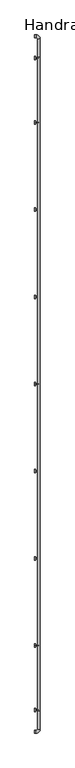
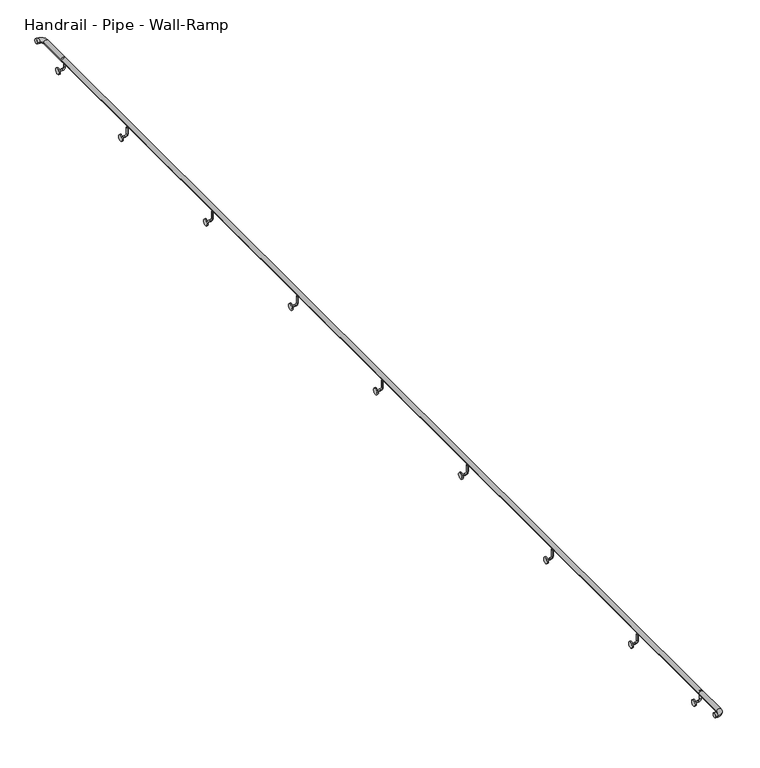
"""IFC4 building model written with IfcOpenShell, lengths in millimetres: railing geometry, Handrail - Pipe - Wall-Ramp."""

from ifc_helpers import new_model, si_unit, point, frame, frame_2d, origin, place, context, project, spatial, circle_curve, ellipse_curve, trimmed, segment, composite_curve, outline, extrude, source, transform, mapped, element, save
from ifc_brep_helpers import plane_surface, cylinder_surface, revolved_surface, advanced_brep


def handrail_pipe_wall_ramp_f1563d15(model_context):
    return source(origin(), model_context, "Body", "SolidModel", [
        extrude(outline(composite_curve([segment(trimmed(circle_curve(frame_2d((895.35, -6025.1478678)), 19.05), [point((895.35, -6006.0978678))], [point((895.35, -6044.1978678))], False, "CARTESIAN"), True, "CONTINUOUS"), segment(trimmed(circle_curve(frame_2d((895.35, -6025.1478678)), 19.05), [point((895.35, -6044.1978678))], [point((895.35, -6006.0978678))], False, "CARTESIAN"), True, "CONTINUOUS")], self_intersect=False)), frame((0.0, -14489.4143828, 0.0), z_axis=(0.0, 1.0, 0.0), x_axis=(0.0, 0.0, 1.0)), (0.0, 0.0, 1.0), 9144.0),
        advanced_brep(
        [(-6025.1478678, -13568.6643828, 857.25), (-6025.1478678, -13581.3643828, 857.25), (-6025.1478678, -13568.6643828, 800.1), (-6025.1478678, -13581.3643828, 800.1), (-6044.1978678, -13581.3643828, 781.05), (-6044.1978678, -13568.6643828, 781.05), (-6072.7728678, -13568.6643828, 781.05), (-6072.7728678, -13581.3643828, 781.05)],
        [
            (0, 1, circle_curve(frame((-6025.1478678, -13575.0143828, 857.25), z_axis=(0.0, 0.0, 1.0), x_axis=(0.0, -1.0, 0.0)), 6.35)),
            (1, 0, circle_curve(frame((-6025.1478678, -13575.0143828, 857.25), z_axis=(0.0, 0.0, 1.0), x_axis=(0.0, -1.0, 0.0)), 6.35)),
            (0, 2),
            (2, 3, circle_curve(frame((-6025.1478678, -13575.0143828, 800.1), z_axis=(0.0, 0.0, 1.0), x_axis=(0.0, -1.0, 0.0)), 6.35)),
            (3, 1),
            (3, 2, circle_curve(frame((-6025.1478678, -13575.0143828, 800.1), z_axis=(0.0, 0.0, 1.0), x_axis=(0.0, -1.0, 0.0)), 6.35)),
            (4, 3, circle_curve(frame((-6044.1978678, -13581.3643828, 800.1), z_axis=(0.0, -1.0, 0.0), x_axis=(1.0, 0.0, 0.0)), 19.05)),
            (2, 5, circle_curve(frame((-6044.1978678, -13568.6643828, 800.1), z_axis=(0.0, 1.0, 0.0), x_axis=(1.0, 0.0, 0.0)), 19.05)),
            (5, 4, circle_curve(frame((-6044.1978678, -13575.0143828, 781.05), z_axis=(1.0, 0.0, 0.0), x_axis=(0.0, -1.0, 0.0)), 6.35)),
            (4, 5, circle_curve(frame((-6044.1978678, -13575.0143828, 781.05), z_axis=(1.0, 0.0, 0.0), x_axis=(0.0, -1.0, 0.0)), 6.35)),
            (6, 7, circle_curve(frame((-6072.7728678, -13575.0143828, 781.05), z_axis=(-1.0, 0.0, 0.0), x_axis=(0.0, -1.0, 0.0)), 6.35)),
            (7, 6, circle_curve(frame((-6072.7728678, -13575.0143828, 781.05), z_axis=(-1.0, 0.0, 0.0), x_axis=(0.0, -1.0, 0.0)), 6.35)),
            (5, 6),
            (7, 4),
        ],
        [
            plane_surface(frame((-6025.1478678, -13581.3643828, 857.25), z_axis=(0.0, 0.0, 1.0), x_axis=(-1.0, 0.0, 0.0))),
            cylinder_surface(frame((-6025.1478678, -13575.0143828, 857.25), z_axis=(0.0, 0.0, 1.0), x_axis=(0.0, -1.0, 0.0)), 6.35),
            revolved_surface(trimmed(ellipse_curve(frame((-6025.1478678, -13575.0143828, 800.1), z_axis=(0.0, 0.0, 1.0), x_axis=(0.0, -1.0, 0.0)), 6.35, 6.35), [point((-6025.1478678, -13568.6643828, 800.1))], [point((-6025.1478678, -13581.3643828, 800.1))], True, "CARTESIAN"), (-6044.1978678, -13575.0143828, 800.1), (0.0, 1.0, 0.0)),
            revolved_surface(trimmed(ellipse_curve(frame((-6025.1478678, -13575.0143828, 800.1), z_axis=(0.0, 0.0, 1.0), x_axis=(0.0, -1.0, 0.0)), 6.35, 6.35), [point((-6025.1478678, -13581.3643828, 800.1))], [point((-6025.1478678, -13568.6643828, 800.1))], True, "CARTESIAN"), (-6044.1978678, -13575.0143828, 800.1), (0.0, 1.0, 0.0)),
            plane_surface(frame((-6072.7728678, -13575.0143828, 774.7), z_axis=(-1.0, 0.0, 0.0), x_axis=(0.0, -1.0, 0.0))),
            cylinder_surface(frame((-6044.1978678, -13575.0143828, 781.05), z_axis=(1.0, 0.0, 0.0), x_axis=(0.0, -1.0, 0.0)), 6.35),
        ],
        [
            (0, [[1, 2]]),
            (1, [[-1, 3, 4, 5]]),
            (1, [[-2, -5, 6, -3]]),
            (2, [[7, -4, 8, 9]]),
            (3, [[-8, -6, -7, 10]]),
            (4, [[11, 12]]),
            (5, [[-9, 13, -12, 14]]),
            (5, [[-10, -14, -11, -13]]),
        ],
    ),
        extrude(outline(composite_curve([segment(trimmed(circle_curve(frame_2d((-13575.0143828, 781.05)), 25.4), [point((-13600.4143828, 781.05))], [point((-13549.6143828, 781.05))], False, "CARTESIAN"), True, "CONTINUOUS"), segment(trimmed(circle_curve(frame_2d((-13575.0143828, 781.05)), 25.4), [point((-13549.6143828, 781.05))], [point((-13600.4143828, 781.05))], False, "CARTESIAN"), True, "CONTINUOUS")], self_intersect=False)), frame((-6082.2978678, 0.0, 0.0), z_axis=(1.0, 0.0, 0.0), x_axis=(0.0, 1.0, 0.0)), (0.0, 0.0, 1.0), 9.525),
        advanced_brep(
        [(-6025.1478678, -12349.4643828, 857.25), (-6025.1478678, -12362.1643828, 857.25), (-6025.1478678, -12349.4643828, 800.1), (-6025.1478678, -12362.1643828, 800.1), (-6044.1978678, -12362.1643828, 781.05), (-6044.1978678, -12349.4643828, 781.05), (-6072.7728678, -12349.4643828, 781.05), (-6072.7728678, -12362.1643828, 781.05)],
        [
            (0, 1, circle_curve(frame((-6025.1478678, -12355.8143828, 857.25), z_axis=(0.0, 0.0, 1.0), x_axis=(0.0, -1.0, 0.0)), 6.35)),
            (1, 0, circle_curve(frame((-6025.1478678, -12355.8143828, 857.25), z_axis=(0.0, 0.0, 1.0), x_axis=(0.0, -1.0, 0.0)), 6.35)),
            (0, 2),
            (2, 3, circle_curve(frame((-6025.1478678, -12355.8143828, 800.1), z_axis=(0.0, 0.0, 1.0), x_axis=(0.0, -1.0, 0.0)), 6.35)),
            (3, 1),
            (3, 2, circle_curve(frame((-6025.1478678, -12355.8143828, 800.1), z_axis=(0.0, 0.0, 1.0), x_axis=(0.0, -1.0, 0.0)), 6.35)),
            (4, 3, circle_curve(frame((-6044.1978678, -12362.1643828, 800.1), z_axis=(0.0, -1.0, 0.0), x_axis=(1.0, 0.0, 0.0)), 19.05)),
            (2, 5, circle_curve(frame((-6044.1978678, -12349.4643828, 800.1), z_axis=(0.0, 1.0, 0.0), x_axis=(1.0, 0.0, 0.0)), 19.05)),
            (5, 4, circle_curve(frame((-6044.1978678, -12355.8143828, 781.05), z_axis=(1.0, 0.0, 0.0), x_axis=(0.0, -1.0, 0.0)), 6.35)),
            (4, 5, circle_curve(frame((-6044.1978678, -12355.8143828, 781.05), z_axis=(1.0, 0.0, 0.0), x_axis=(0.0, -1.0, 0.0)), 6.35)),
            (6, 7, circle_curve(frame((-6072.7728678, -12355.8143828, 781.05), z_axis=(-1.0, 0.0, 0.0), x_axis=(0.0, -1.0, 0.0)), 6.35)),
            (7, 6, circle_curve(frame((-6072.7728678, -12355.8143828, 781.05), z_axis=(-1.0, 0.0, 0.0), x_axis=(0.0, -1.0, 0.0)), 6.35)),
            (5, 6),
            (7, 4),
        ],
        [
            plane_surface(frame((-6025.1478678, -12362.1643828, 857.25), z_axis=(0.0, 0.0, 1.0), x_axis=(-1.0, 0.0, 0.0))),
            cylinder_surface(frame((-6025.1478678, -12355.8143828, 857.25), z_axis=(0.0, 0.0, 1.0), x_axis=(0.0, -1.0, 0.0)), 6.35),
            revolved_surface(trimmed(ellipse_curve(frame((-6025.1478678, -12355.8143828, 800.1), z_axis=(0.0, 0.0, 1.0), x_axis=(0.0, -1.0, 0.0)), 6.35, 6.35), [point((-6025.1478678, -12349.4643828, 800.1))], [point((-6025.1478678, -12362.1643828, 800.1))], True, "CARTESIAN"), (-6044.1978678, -12355.8143828, 800.1), (0.0, 1.0, 0.0)),
            revolved_surface(trimmed(ellipse_curve(frame((-6025.1478678, -12355.8143828, 800.1), z_axis=(0.0, 0.0, 1.0), x_axis=(0.0, -1.0, 0.0)), 6.35, 6.35), [point((-6025.1478678, -12362.1643828, 800.1))], [point((-6025.1478678, -12349.4643828, 800.1))], True, "CARTESIAN"), (-6044.1978678, -12355.8143828, 800.1), (0.0, 1.0, 0.0)),
            plane_surface(frame((-6072.7728678, -12355.8143828, 774.7), z_axis=(-1.0, 0.0, 0.0), x_axis=(0.0, -1.0, 0.0))),
            cylinder_surface(frame((-6044.1978678, -12355.8143828, 781.05), z_axis=(1.0, 0.0, 0.0), x_axis=(0.0, -1.0, 0.0)), 6.35),
        ],
        [
            (0, [[1, 2]]),
            (1, [[-1, 3, 4, 5]]),
            (1, [[-2, -5, 6, -3]]),
            (2, [[7, -4, 8, 9]]),
            (3, [[-8, -6, -7, 10]]),
            (4, [[11, 12]]),
            (5, [[-9, 13, -12, 14]]),
            (5, [[-10, -14, -11, -13]]),
        ],
    ),
        extrude(outline(composite_curve([segment(trimmed(circle_curve(frame_2d((-12355.8143828, 781.05)), 25.4), [point((-12381.2143828, 781.05))], [point((-12330.4143828, 781.05))], False, "CARTESIAN"), True, "CONTINUOUS"), segment(trimmed(circle_curve(frame_2d((-12355.8143828, 781.05)), 25.4), [point((-12330.4143828, 781.05))], [point((-12381.2143828, 781.05))], False, "CARTESIAN"), True, "CONTINUOUS")], self_intersect=False)), frame((-6082.2978678, 0.0, 0.0), z_axis=(1.0, 0.0, 0.0), x_axis=(0.0, 1.0, 0.0)), (0.0, 0.0, 1.0), 9.525),
        advanced_brep(
        [(-6025.1478678, -11130.2643828, 857.25), (-6025.1478678, -11142.9643828, 857.25), (-6025.1478678, -11130.2643828, 800.1), (-6025.1478678, -11142.9643828, 800.1), (-6044.1978678, -11142.9643828, 781.05), (-6044.1978678, -11130.2643828, 781.05), (-6072.7728678, -11130.2643828, 781.05), (-6072.7728678, -11142.9643828, 781.05)],
        [
            (0, 1, circle_curve(frame((-6025.1478678, -11136.6143828, 857.25), z_axis=(0.0, 0.0, 1.0), x_axis=(0.0, -1.0, 0.0)), 6.35)),
            (1, 0, circle_curve(frame((-6025.1478678, -11136.6143828, 857.25), z_axis=(0.0, 0.0, 1.0), x_axis=(0.0, -1.0, 0.0)), 6.35)),
            (0, 2),
            (2, 3, circle_curve(frame((-6025.1478678, -11136.6143828, 800.1), z_axis=(0.0, 0.0, 1.0), x_axis=(0.0, -1.0, 0.0)), 6.35)),
            (3, 1),
            (3, 2, circle_curve(frame((-6025.1478678, -11136.6143828, 800.1), z_axis=(0.0, 0.0, 1.0), x_axis=(0.0, -1.0, 0.0)), 6.35)),
            (4, 3, circle_curve(frame((-6044.1978678, -11142.9643828, 800.1), z_axis=(0.0, -1.0, 0.0), x_axis=(1.0, 0.0, 0.0)), 19.05)),
            (2, 5, circle_curve(frame((-6044.1978678, -11130.2643828, 800.1), z_axis=(0.0, 1.0, 0.0), x_axis=(1.0, 0.0, 0.0)), 19.05)),
            (5, 4, circle_curve(frame((-6044.1978678, -11136.6143828, 781.05), z_axis=(1.0, 0.0, 0.0), x_axis=(0.0, -1.0, 0.0)), 6.35)),
            (4, 5, circle_curve(frame((-6044.1978678, -11136.6143828, 781.05), z_axis=(1.0, 0.0, 0.0), x_axis=(0.0, -1.0, 0.0)), 6.35)),
            (6, 7, circle_curve(frame((-6072.7728678, -11136.6143828, 781.05), z_axis=(-1.0, 0.0, 0.0), x_axis=(0.0, -1.0, 0.0)), 6.35)),
            (7, 6, circle_curve(frame((-6072.7728678, -11136.6143828, 781.05), z_axis=(-1.0, 0.0, 0.0), x_axis=(0.0, -1.0, 0.0)), 6.35)),
            (5, 6),
            (7, 4),
        ],
        [
            plane_surface(frame((-6025.1478678, -11142.9643828, 857.25), z_axis=(0.0, 0.0, 1.0), x_axis=(-1.0, 0.0, 0.0))),
            cylinder_surface(frame((-6025.1478678, -11136.6143828, 857.25), z_axis=(0.0, 0.0, 1.0), x_axis=(0.0, -1.0, 0.0)), 6.35),
            revolved_surface(trimmed(ellipse_curve(frame((-6025.1478678, -11136.6143828, 800.1), z_axis=(0.0, 0.0, 1.0), x_axis=(0.0, -1.0, 0.0)), 6.35, 6.35), [point((-6025.1478678, -11130.2643828, 800.1))], [point((-6025.1478678, -11142.9643828, 800.1))], True, "CARTESIAN"), (-6044.1978678, -11136.6143828, 800.1), (0.0, 1.0, 0.0)),
            revolved_surface(trimmed(ellipse_curve(frame((-6025.1478678, -11136.6143828, 800.1), z_axis=(0.0, 0.0, 1.0), x_axis=(0.0, -1.0, 0.0)), 6.35, 6.35), [point((-6025.1478678, -11142.9643828, 800.1))], [point((-6025.1478678, -11130.2643828, 800.1))], True, "CARTESIAN"), (-6044.1978678, -11136.6143828, 800.1), (0.0, 1.0, 0.0)),
            plane_surface(frame((-6072.7728678, -11136.6143828, 774.7), z_axis=(-1.0, 0.0, 0.0), x_axis=(0.0, -1.0, 0.0))),
            cylinder_surface(frame((-6044.1978678, -11136.6143828, 781.05), z_axis=(1.0, 0.0, 0.0), x_axis=(0.0, -1.0, 0.0)), 6.35),
        ],
        [
            (0, [[1, 2]]),
            (1, [[-1, 3, 4, 5]]),
            (1, [[-2, -5, 6, -3]]),
            (2, [[7, -4, 8, 9]]),
            (3, [[-8, -6, -7, 10]]),
            (4, [[11, 12]]),
            (5, [[-9, 13, -12, 14]]),
            (5, [[-10, -14, -11, -13]]),
        ],
    ),
        extrude(outline(composite_curve([segment(trimmed(circle_curve(frame_2d((-11136.6143828, 781.05)), 25.4), [point((-11162.0143828, 781.05))], [point((-11111.2143828, 781.05))], False, "CARTESIAN"), True, "CONTINUOUS"), segment(trimmed(circle_curve(frame_2d((-11136.6143828, 781.05)), 25.4), [point((-11111.2143828, 781.05))], [point((-11162.0143828, 781.05))], False, "CARTESIAN"), True, "CONTINUOUS")], self_intersect=False)), frame((-6082.2978678, 0.0, 0.0), z_axis=(1.0, 0.0, 0.0), x_axis=(0.0, 1.0, 0.0)), (0.0, 0.0, 1.0), 9.525),
        advanced_brep(
        [(-6025.1478678, -9911.0643828, 857.25), (-6025.1478678, -9923.7643828, 857.25), (-6025.1478678, -9911.0643828, 800.1), (-6025.1478678, -9923.7643828, 800.1), (-6044.1978678, -9923.7643828, 781.05), (-6044.1978678, -9911.0643828, 781.05), (-6072.7728678, -9911.0643828, 781.05), (-6072.7728678, -9923.7643828, 781.05)],
        [
            (0, 1, circle_curve(frame((-6025.1478678, -9917.4143828, 857.25), z_axis=(0.0, 0.0, 1.0), x_axis=(0.0, -1.0, 0.0)), 6.35)),
            (1, 0, circle_curve(frame((-6025.1478678, -9917.4143828, 857.25), z_axis=(0.0, 0.0, 1.0), x_axis=(0.0, -1.0, 0.0)), 6.35)),
            (0, 2),
            (2, 3, circle_curve(frame((-6025.1478678, -9917.4143828, 800.1), z_axis=(0.0, 0.0, 1.0), x_axis=(0.0, -1.0, 0.0)), 6.35)),
            (3, 1),
            (3, 2, circle_curve(frame((-6025.1478678, -9917.4143828, 800.1), z_axis=(0.0, 0.0, 1.0), x_axis=(0.0, -1.0, 0.0)), 6.35)),
            (4, 3, circle_curve(frame((-6044.1978678, -9923.7643828, 800.1), z_axis=(0.0, -1.0, 0.0), x_axis=(1.0, 0.0, 0.0)), 19.05)),
            (2, 5, circle_curve(frame((-6044.1978678, -9911.0643828, 800.1), z_axis=(0.0, 1.0, 0.0), x_axis=(1.0, 0.0, 0.0)), 19.05)),
            (5, 4, circle_curve(frame((-6044.1978678, -9917.4143828, 781.05), z_axis=(1.0, 0.0, 0.0), x_axis=(0.0, -1.0, 0.0)), 6.35)),
            (4, 5, circle_curve(frame((-6044.1978678, -9917.4143828, 781.05), z_axis=(1.0, 0.0, 0.0), x_axis=(0.0, -1.0, 0.0)), 6.35)),
            (6, 7, circle_curve(frame((-6072.7728678, -9917.4143828, 781.05), z_axis=(-1.0, 0.0, 0.0), x_axis=(0.0, -1.0, 0.0)), 6.35)),
            (7, 6, circle_curve(frame((-6072.7728678, -9917.4143828, 781.05), z_axis=(-1.0, 0.0, 0.0), x_axis=(0.0, -1.0, 0.0)), 6.35)),
            (5, 6),
            (7, 4),
        ],
        [
            plane_surface(frame((-6025.1478678, -9923.7643828, 857.25), z_axis=(0.0, 0.0, 1.0), x_axis=(-1.0, 0.0, 0.0))),
            cylinder_surface(frame((-6025.1478678, -9917.4143828, 857.25), z_axis=(0.0, 0.0, 1.0), x_axis=(0.0, -1.0, 0.0)), 6.35),
            revolved_surface(trimmed(ellipse_curve(frame((-6025.1478678, -9917.4143828, 800.1), z_axis=(0.0, 0.0, 1.0), x_axis=(0.0, -1.0, 0.0)), 6.35, 6.35), [point((-6025.1478678, -9911.0643828, 800.1))], [point((-6025.1478678, -9923.7643828, 800.1))], True, "CARTESIAN"), (-6044.1978678, -9917.4143828, 800.1), (0.0, 1.0, 0.0)),
            revolved_surface(trimmed(ellipse_curve(frame((-6025.1478678, -9917.4143828, 800.1), z_axis=(0.0, 0.0, 1.0), x_axis=(0.0, -1.0, 0.0)), 6.35, 6.35), [point((-6025.1478678, -9923.7643828, 800.1))], [point((-6025.1478678, -9911.0643828, 800.1))], True, "CARTESIAN"), (-6044.1978678, -9917.4143828, 800.1), (0.0, 1.0, 0.0)),
            plane_surface(frame((-6072.7728678, -9917.4143828, 774.7), z_axis=(-1.0, 0.0, 0.0), x_axis=(0.0, -1.0, 0.0))),
            cylinder_surface(frame((-6044.1978678, -9917.4143828, 781.05), z_axis=(1.0, 0.0, 0.0), x_axis=(0.0, -1.0, 0.0)), 6.35),
        ],
        [
            (0, [[1, 2]]),
            (1, [[-1, 3, 4, 5]]),
            (1, [[-2, -5, 6, -3]]),
            (2, [[7, -4, 8, 9]]),
            (3, [[-8, -6, -7, 10]]),
            (4, [[11, 12]]),
            (5, [[-9, 13, -12, 14]]),
            (5, [[-10, -14, -11, -13]]),
        ],
    ),
        extrude(outline(composite_curve([segment(trimmed(circle_curve(frame_2d((-9917.4143828, 781.05)), 25.4), [point((-9942.8143828, 781.05))], [point((-9892.0143828, 781.05))], False, "CARTESIAN"), True, "CONTINUOUS"), segment(trimmed(circle_curve(frame_2d((-9917.4143828, 781.05)), 25.4), [point((-9892.0143828, 781.05))], [point((-9942.8143828, 781.05))], False, "CARTESIAN"), True, "CONTINUOUS")], self_intersect=False)), frame((-6082.2978678, 0.0, 0.0), z_axis=(1.0, 0.0, 0.0), x_axis=(0.0, 1.0, 0.0)), (0.0, 0.0, 1.0), 9.525),
        advanced_brep(
        [(-6025.1478678, -8691.8643828, 857.25), (-6025.1478678, -8704.5643828, 857.25), (-6025.1478678, -8691.8643828, 800.1), (-6025.1478678, -8704.5643828, 800.1), (-6044.1978678, -8704.5643828, 781.05), (-6044.1978678, -8691.8643828, 781.05), (-6072.7728678, -8691.8643828, 781.05), (-6072.7728678, -8704.5643828, 781.05)],
        [
            (0, 1, circle_curve(frame((-6025.1478678, -8698.2143828, 857.25), z_axis=(0.0, 0.0, 1.0), x_axis=(0.0, -1.0, 0.0)), 6.35)),
            (1, 0, circle_curve(frame((-6025.1478678, -8698.2143828, 857.25), z_axis=(0.0, 0.0, 1.0), x_axis=(0.0, -1.0, 0.0)), 6.35)),
            (0, 2),
            (2, 3, circle_curve(frame((-6025.1478678, -8698.2143828, 800.1), z_axis=(0.0, 0.0, 1.0), x_axis=(0.0, -1.0, 0.0)), 6.35)),
            (3, 1),
            (3, 2, circle_curve(frame((-6025.1478678, -8698.2143828, 800.1), z_axis=(0.0, 0.0, 1.0), x_axis=(0.0, -1.0, 0.0)), 6.35)),
            (4, 3, circle_curve(frame((-6044.1978678, -8704.5643828, 800.1), z_axis=(0.0, -1.0, 0.0), x_axis=(1.0, 0.0, 0.0)), 19.05)),
            (2, 5, circle_curve(frame((-6044.1978678, -8691.8643828, 800.1), z_axis=(0.0, 1.0, 0.0), x_axis=(1.0, 0.0, 0.0)), 19.05)),
            (5, 4, circle_curve(frame((-6044.1978678, -8698.2143828, 781.05), z_axis=(1.0, 0.0, 0.0), x_axis=(0.0, -1.0, 0.0)), 6.35)),
            (4, 5, circle_curve(frame((-6044.1978678, -8698.2143828, 781.05), z_axis=(1.0, 0.0, 0.0), x_axis=(0.0, -1.0, 0.0)), 6.35)),
            (6, 7, circle_curve(frame((-6072.7728678, -8698.2143828, 781.05), z_axis=(-1.0, 0.0, 0.0), x_axis=(0.0, -1.0, 0.0)), 6.35)),
            (7, 6, circle_curve(frame((-6072.7728678, -8698.2143828, 781.05), z_axis=(-1.0, 0.0, 0.0), x_axis=(0.0, -1.0, 0.0)), 6.35)),
            (5, 6),
            (7, 4),
        ],
        [
            plane_surface(frame((-6025.1478678, -8704.5643828, 857.25), z_axis=(0.0, 0.0, 1.0), x_axis=(-1.0, 0.0, 0.0))),
            cylinder_surface(frame((-6025.1478678, -8698.2143828, 857.25), z_axis=(0.0, 0.0, 1.0), x_axis=(0.0, -1.0, 0.0)), 6.35),
            revolved_surface(trimmed(ellipse_curve(frame((-6025.1478678, -8698.2143828, 800.1), z_axis=(0.0, 0.0, 1.0), x_axis=(0.0, -1.0, 0.0)), 6.35, 6.35), [point((-6025.1478678, -8691.8643828, 800.1))], [point((-6025.1478678, -8704.5643828, 800.1))], True, "CARTESIAN"), (-6044.1978678, -8698.2143828, 800.1), (0.0, 1.0, 0.0)),
            revolved_surface(trimmed(ellipse_curve(frame((-6025.1478678, -8698.2143828, 800.1), z_axis=(0.0, 0.0, 1.0), x_axis=(0.0, -1.0, 0.0)), 6.35, 6.35), [point((-6025.1478678, -8704.5643828, 800.1))], [point((-6025.1478678, -8691.8643828, 800.1))], True, "CARTESIAN"), (-6044.1978678, -8698.2143828, 800.1), (0.0, 1.0, 0.0)),
            plane_surface(frame((-6072.7728678, -8698.2143828, 774.7), z_axis=(-1.0, 0.0, 0.0), x_axis=(0.0, -1.0, 0.0))),
            cylinder_surface(frame((-6044.1978678, -8698.2143828, 781.05), z_axis=(1.0, 0.0, 0.0), x_axis=(0.0, -1.0, 0.0)), 6.35),
        ],
        [
            (0, [[1, 2]]),
            (1, [[-1, 3, 4, 5]]),
            (1, [[-2, -5, 6, -3]]),
            (2, [[7, -4, 8, 9]]),
            (3, [[-8, -6, -7, 10]]),
            (4, [[11, 12]]),
            (5, [[-9, 13, -12, 14]]),
            (5, [[-10, -14, -11, -13]]),
        ],
    ),
        extrude(outline(composite_curve([segment(trimmed(circle_curve(frame_2d((-8698.2143828, 781.05)), 25.4), [point((-8723.6143828, 781.05))], [point((-8672.8143828, 781.05))], False, "CARTESIAN"), True, "CONTINUOUS"), segment(trimmed(circle_curve(frame_2d((-8698.2143828, 781.05)), 25.4), [point((-8672.8143828, 781.05))], [point((-8723.6143828, 781.05))], False, "CARTESIAN"), True, "CONTINUOUS")], self_intersect=False)), frame((-6082.2978678, 0.0, 0.0), z_axis=(1.0, 0.0, 0.0), x_axis=(0.0, 1.0, 0.0)), (0.0, 0.0, 1.0), 9.525),
        advanced_brep(
        [(-6025.1478678, -7472.6643828, 857.25), (-6025.1478678, -7485.3643828, 857.25), (-6025.1478678, -7472.6643828, 800.1), (-6025.1478678, -7485.3643828, 800.1), (-6044.1978678, -7485.3643828, 781.05), (-6044.1978678, -7472.6643828, 781.05), (-6072.7728678, -7472.6643828, 781.05), (-6072.7728678, -7485.3643828, 781.05)],
        [
            (0, 1, circle_curve(frame((-6025.1478678, -7479.0143828, 857.25), z_axis=(0.0, 0.0, 1.0), x_axis=(0.0, -1.0, 0.0)), 6.35)),
            (1, 0, circle_curve(frame((-6025.1478678, -7479.0143828, 857.25), z_axis=(0.0, 0.0, 1.0), x_axis=(0.0, -1.0, 0.0)), 6.35)),
            (0, 2),
            (2, 3, circle_curve(frame((-6025.1478678, -7479.0143828, 800.1), z_axis=(0.0, 0.0, 1.0), x_axis=(0.0, -1.0, 0.0)), 6.35)),
            (3, 1),
            (3, 2, circle_curve(frame((-6025.1478678, -7479.0143828, 800.1), z_axis=(0.0, 0.0, 1.0), x_axis=(0.0, -1.0, 0.0)), 6.35)),
            (4, 3, circle_curve(frame((-6044.1978678, -7485.3643828, 800.1), z_axis=(0.0, -1.0, 0.0), x_axis=(1.0, 0.0, 0.0)), 19.05)),
            (2, 5, circle_curve(frame((-6044.1978678, -7472.6643828, 800.1), z_axis=(0.0, 1.0, 0.0), x_axis=(1.0, 0.0, 0.0)), 19.05)),
            (5, 4, circle_curve(frame((-6044.1978678, -7479.0143828, 781.05), z_axis=(1.0, 0.0, 0.0), x_axis=(0.0, -1.0, 0.0)), 6.35)),
            (4, 5, circle_curve(frame((-6044.1978678, -7479.0143828, 781.05), z_axis=(1.0, 0.0, 0.0), x_axis=(0.0, -1.0, 0.0)), 6.35)),
            (6, 7, circle_curve(frame((-6072.7728678, -7479.0143828, 781.05), z_axis=(-1.0, 0.0, 0.0), x_axis=(0.0, -1.0, 0.0)), 6.35)),
            (7, 6, circle_curve(frame((-6072.7728678, -7479.0143828, 781.05), z_axis=(-1.0, 0.0, 0.0), x_axis=(0.0, -1.0, 0.0)), 6.35)),
            (5, 6),
            (7, 4),
        ],
        [
            plane_surface(frame((-6025.1478678, -7485.3643828, 857.25), z_axis=(0.0, 0.0, 1.0), x_axis=(-1.0, 0.0, 0.0))),
            cylinder_surface(frame((-6025.1478678, -7479.0143828, 857.25), z_axis=(0.0, 0.0, 1.0), x_axis=(0.0, -1.0, 0.0)), 6.35),
            revolved_surface(trimmed(ellipse_curve(frame((-6025.1478678, -7479.0143828, 800.1), z_axis=(0.0, 0.0, 1.0), x_axis=(0.0, -1.0, 0.0)), 6.35, 6.35), [point((-6025.1478678, -7472.6643828, 800.1))], [point((-6025.1478678, -7485.3643828, 800.1))], True, "CARTESIAN"), (-6044.1978678, -7479.0143828, 800.1), (0.0, 1.0, 0.0)),
            revolved_surface(trimmed(ellipse_curve(frame((-6025.1478678, -7479.0143828, 800.1), z_axis=(0.0, 0.0, 1.0), x_axis=(0.0, -1.0, 0.0)), 6.35, 6.35), [point((-6025.1478678, -7485.3643828, 800.1))], [point((-6025.1478678, -7472.6643828, 800.1))], True, "CARTESIAN"), (-6044.1978678, -7479.0143828, 800.1), (0.0, 1.0, 0.0)),
            plane_surface(frame((-6072.7728678, -7479.0143828, 774.7), z_axis=(-1.0, 0.0, 0.0), x_axis=(0.0, -1.0, 0.0))),
            cylinder_surface(frame((-6044.1978678, -7479.0143828, 781.05), z_axis=(1.0, 0.0, 0.0), x_axis=(0.0, -1.0, 0.0)), 6.35),
        ],
        [
            (0, [[1, 2]]),
            (1, [[-1, 3, 4, 5]]),
            (1, [[-2, -5, 6, -3]]),
            (2, [[7, -4, 8, 9]]),
            (3, [[-8, -6, -7, 10]]),
            (4, [[11, 12]]),
            (5, [[-9, 13, -12, 14]]),
            (5, [[-10, -14, -11, -13]]),
        ],
    ),
        extrude(outline(composite_curve([segment(trimmed(circle_curve(frame_2d((-7479.0143828, 781.05)), 25.4), [point((-7504.4143828, 781.05))], [point((-7453.6143828, 781.05))], False, "CARTESIAN"), True, "CONTINUOUS"), segment(trimmed(circle_curve(frame_2d((-7479.0143828, 781.05)), 25.4), [point((-7453.6143828, 781.05))], [point((-7504.4143828, 781.05))], False, "CARTESIAN"), True, "CONTINUOUS")], self_intersect=False)), frame((-6082.2978678, 0.0, 0.0), z_axis=(1.0, 0.0, 0.0), x_axis=(0.0, 1.0, 0.0)), (0.0, 0.0, 1.0), 9.525),
        advanced_brep(
        [(-6025.1478678, -6253.4643828, 857.25), (-6025.1478678, -6266.1643828, 857.25), (-6025.1478678, -6253.4643828, 800.1), (-6025.1478678, -6266.1643828, 800.1), (-6044.1978678, -6266.1643828, 781.05), (-6044.1978678, -6253.4643828, 781.05), (-6072.7728678, -6253.4643828, 781.05), (-6072.7728678, -6266.1643828, 781.05)],
        [
            (0, 1, circle_curve(frame((-6025.1478678, -6259.8143828, 857.25), z_axis=(0.0, 0.0, 1.0), x_axis=(0.0, -1.0, 0.0)), 6.35)),
            (1, 0, circle_curve(frame((-6025.1478678, -6259.8143828, 857.25), z_axis=(0.0, 0.0, 1.0), x_axis=(0.0, -1.0, 0.0)), 6.35)),
            (0, 2),
            (2, 3, circle_curve(frame((-6025.1478678, -6259.8143828, 800.1), z_axis=(0.0, 0.0, 1.0), x_axis=(0.0, -1.0, 0.0)), 6.35)),
            (3, 1),
            (3, 2, circle_curve(frame((-6025.1478678, -6259.8143828, 800.1), z_axis=(0.0, 0.0, 1.0), x_axis=(0.0, -1.0, 0.0)), 6.35)),
            (4, 3, circle_curve(frame((-6044.1978678, -6266.1643828, 800.1), z_axis=(0.0, -1.0, 0.0), x_axis=(1.0, 0.0, 0.0)), 19.05)),
            (2, 5, circle_curve(frame((-6044.1978678, -6253.4643828, 800.1), z_axis=(0.0, 1.0, 0.0), x_axis=(1.0, 0.0, 0.0)), 19.05)),
            (5, 4, circle_curve(frame((-6044.1978678, -6259.8143828, 781.05), z_axis=(1.0, 0.0, 0.0), x_axis=(0.0, -1.0, 0.0)), 6.35)),
            (4, 5, circle_curve(frame((-6044.1978678, -6259.8143828, 781.05), z_axis=(1.0, 0.0, 0.0), x_axis=(0.0, -1.0, 0.0)), 6.35)),
            (6, 7, circle_curve(frame((-6072.7728678, -6259.8143828, 781.05), z_axis=(-1.0, 0.0, 0.0), x_axis=(0.0, -1.0, 0.0)), 6.35)),
            (7, 6, circle_curve(frame((-6072.7728678, -6259.8143828, 781.05), z_axis=(-1.0, 0.0, 0.0), x_axis=(0.0, -1.0, 0.0)), 6.35)),
            (5, 6),
            (7, 4),
        ],
        [
            plane_surface(frame((-6025.1478678, -6266.1643828, 857.25), z_axis=(0.0, 0.0, 1.0), x_axis=(-1.0, 0.0, 0.0))),
            cylinder_surface(frame((-6025.1478678, -6259.8143828, 857.25), z_axis=(0.0, 0.0, 1.0), x_axis=(0.0, -1.0, 0.0)), 6.35),
            revolved_surface(trimmed(ellipse_curve(frame((-6025.1478678, -6259.8143828, 800.1), z_axis=(0.0, 0.0, 1.0), x_axis=(0.0, -1.0, 0.0)), 6.35, 6.35), [point((-6025.1478678, -6253.4643828, 800.1))], [point((-6025.1478678, -6266.1643828, 800.1))], True, "CARTESIAN"), (-6044.1978678, -6259.8143828, 800.1), (0.0, 1.0, 0.0)),
            revolved_surface(trimmed(ellipse_curve(frame((-6025.1478678, -6259.8143828, 800.1), z_axis=(0.0, 0.0, 1.0), x_axis=(0.0, -1.0, 0.0)), 6.35, 6.35), [point((-6025.1478678, -6266.1643828, 800.1))], [point((-6025.1478678, -6253.4643828, 800.1))], True, "CARTESIAN"), (-6044.1978678, -6259.8143828, 800.1), (0.0, 1.0, 0.0)),
            plane_surface(frame((-6072.7728678, -6259.8143828, 774.7), z_axis=(-1.0, 0.0, 0.0), x_axis=(0.0, -1.0, 0.0))),
            cylinder_surface(frame((-6044.1978678, -6259.8143828, 781.05), z_axis=(1.0, 0.0, 0.0), x_axis=(0.0, -1.0, 0.0)), 6.35),
        ],
        [
            (0, [[1, 2]]),
            (1, [[-1, 3, 4, 5]]),
            (1, [[-2, -5, 6, -3]]),
            (2, [[7, -4, 8, 9]]),
            (3, [[-8, -6, -7, 10]]),
            (4, [[11, 12]]),
            (5, [[-9, 13, -12, 14]]),
            (5, [[-10, -14, -11, -13]]),
        ],
    ),
        extrude(outline(composite_curve([segment(trimmed(circle_curve(frame_2d((-6259.8143828, 781.05)), 25.4), [point((-6285.2143828, 781.05))], [point((-6234.4143828, 781.05))], False, "CARTESIAN"), True, "CONTINUOUS"), segment(trimmed(circle_curve(frame_2d((-6259.8143828, 781.05)), 25.4), [point((-6234.4143828, 781.05))], [point((-6285.2143828, 781.05))], False, "CARTESIAN"), True, "CONTINUOUS")], self_intersect=False)), frame((-6082.2978678, 0.0, 0.0), z_axis=(1.0, 0.0, 0.0), x_axis=(0.0, 1.0, 0.0)), (0.0, 0.0, 1.0), 9.525),
        advanced_brep(
        [(-6044.1978678, -14476.7143828, 895.35), (-6006.0978678, -14476.7143828, 895.35), (-6044.1978678, -14743.4143828, 895.35), (-6006.0978678, -14743.4143828, 895.35), (-6063.2478678, -14800.5643828, 895.35), (-6063.2478678, -14762.4643828, 895.35), (-6082.2978678, -14762.4643828, 895.35), (-6082.2978678, -14800.5643828, 895.35)],
        [
            (0, 1, circle_curve(frame((-6025.1478678, -14476.7143828, 895.35), z_axis=(0.0, 1.0, 0.0), x_axis=(1.0, 0.0, 0.0)), 19.05)),
            (1, 0, circle_curve(frame((-6025.1478678, -14476.7143828, 895.35), z_axis=(0.0, 1.0, 0.0), x_axis=(1.0, 0.0, 0.0)), 19.05)),
            (0, 2),
            (2, 3, circle_curve(frame((-6025.1478678, -14743.4143828, 895.35), z_axis=(0.0, 1.0, 0.0), x_axis=(1.0, 0.0, 0.0)), 19.05)),
            (3, 1),
            (3, 2, circle_curve(frame((-6025.1478678, -14743.4143828, 895.35), z_axis=(0.0, 1.0, 0.0), x_axis=(1.0, 0.0, 0.0)), 19.05)),
            (4, 3, circle_curve(frame((-6063.2478678, -14743.4143828, 895.35), z_axis=(0.0, 0.0, 1.0), x_axis=(1.0, 0.0, 0.0)), 57.15)),
            (2, 5, circle_curve(frame((-6063.2478678, -14743.4143828, 895.35), z_axis=(0.0, 0.0, -1.0), x_axis=(1.0, 0.0, 0.0)), 19.05)),
            (5, 4, circle_curve(frame((-6063.2478678, -14781.5143828, 895.35), z_axis=(1.0, 0.0, 0.0), x_axis=(0.0, -1.0, 0.0)), 19.05)),
            (4, 5, circle_curve(frame((-6063.2478678, -14781.5143828, 895.35), z_axis=(1.0, 0.0, 0.0), x_axis=(0.0, -1.0, 0.0)), 19.05)),
            (6, 7, circle_curve(frame((-6082.2978678, -14781.5143828, 895.35), z_axis=(-1.0, 0.0, 0.0), x_axis=(0.0, -1.0, 0.0)), 19.05)),
            (7, 6, circle_curve(frame((-6082.2978678, -14781.5143828, 895.35), z_axis=(-1.0, 0.0, 0.0), x_axis=(0.0, -1.0, 0.0)), 19.05)),
            (5, 6),
            (7, 4),
        ],
        [
            plane_surface(frame((-6025.1478678, -14476.7143828, 895.35), z_axis=(0.0, 1.0, 0.0), x_axis=(0.0, 0.0, 1.0))),
            cylinder_surface(frame((-6025.1478678, -14476.7143828, 895.35), z_axis=(0.0, 1.0, 0.0), x_axis=(1.0, 0.0, 0.0)), 19.05),
            revolved_surface(trimmed(ellipse_curve(frame((-6025.1478678, -14743.4143828, 895.35), z_axis=(0.0, 1.0, 0.0), x_axis=(1.0, 0.0, 0.0)), 19.05, 19.05), [point((-6044.1978678, -14743.4143828, 895.35))], [point((-6006.0978678, -14743.4143828, 895.35))], True, "CARTESIAN"), (-6063.2478678, -14743.4143828, 895.35), (0.0, 0.0, -1.0)),
            revolved_surface(trimmed(ellipse_curve(frame((-6025.1478678, -14743.4143828, 895.35), z_axis=(0.0, 1.0, 0.0), x_axis=(1.0, 0.0, 0.0)), 19.05, 19.05), [point((-6006.0978678, -14743.4143828, 895.35))], [point((-6044.1978678, -14743.4143828, 895.35))], True, "CARTESIAN"), (-6063.2478678, -14743.4143828, 895.35), (0.0, 0.0, -1.0)),
            plane_surface(frame((-6082.2978678, -14781.5143828, 895.35), z_axis=(-1.0, 0.0, 0.0), x_axis=(0.0, 0.0, 1.0))),
            cylinder_surface(frame((-6063.2478678, -14781.5143828, 895.35), z_axis=(1.0, 0.0, 0.0), x_axis=(0.0, -1.0, 0.0)), 19.05),
        ],
        [
            (0, [[1, 2]]),
            (1, [[-1, 3, 4, 5]]),
            (1, [[-2, -5, 6, -3]]),
            (2, [[7, -4, 8, 9]]),
            (3, [[-8, -6, -7, 10]]),
            (4, [[11, 12]]),
            (5, [[-9, 13, -12, 14]]),
            (5, [[-10, -14, -11, -13]]),
        ],
    ),
        advanced_brep(
        [(-6072.7728678, -14476.7143828, 812.8), (-6072.7728678, -14476.7143828, 825.5), (-6044.1978678, -14476.7143828, 812.8), (-6044.1978678, -14476.7143828, 825.5), (-6031.4978678, -14476.7143828, 838.2), (-6018.7978678, -14476.7143828, 838.2), (-6018.7978678, -14476.7143828, 895.35), (-6031.4978678, -14476.7143828, 895.35)],
        [
            (0, 1, circle_curve(frame((-6072.7728678, -14476.7143828, 819.15), z_axis=(-1.0, 0.0, 0.0), x_axis=(0.0, 0.0, 1.0)), 6.35)),
            (1, 0, circle_curve(frame((-6072.7728678, -14476.7143828, 819.15), z_axis=(-1.0, 0.0, 0.0), x_axis=(0.0, 0.0, 1.0)), 6.35)),
            (0, 2),
            (2, 3, circle_curve(frame((-6044.1978678, -14476.7143828, 819.15), z_axis=(-1.0, 0.0, 0.0), x_axis=(0.0, 0.0, 1.0)), 6.35)),
            (3, 1),
            (3, 2, circle_curve(frame((-6044.1978678, -14476.7143828, 819.15), z_axis=(-1.0, 0.0, 0.0), x_axis=(0.0, 0.0, 1.0)), 6.35)),
            (4, 3, circle_curve(frame((-6044.1978678, -14476.7143828, 838.2), z_axis=(0.0, 1.0, 0.0), x_axis=(0.0, 0.0, -1.0)), 12.7)),
            (2, 5, circle_curve(frame((-6044.1978678, -14476.7143828, 838.2), z_axis=(0.0, -1.0, 0.0), x_axis=(0.0, 0.0, -1.0)), 25.4)),
            (5, 4, circle_curve(frame((-6025.1478678, -14476.7143828, 838.2), z_axis=(0.0, 0.0, -1.0), x_axis=(-1.0, 0.0, 0.0)), 6.35)),
            (4, 5, circle_curve(frame((-6025.1478678, -14476.7143828, 838.2), z_axis=(0.0, 0.0, -1.0), x_axis=(-1.0, 0.0, 0.0)), 6.35)),
            (6, 7, circle_curve(frame((-6025.1478678, -14476.7143828, 895.35), z_axis=(0.0, 0.0, 1.0), x_axis=(-1.0, 0.0, 0.0)), 6.35)),
            (7, 6, circle_curve(frame((-6025.1478678, -14476.7143828, 895.35), z_axis=(0.0, 0.0, 1.0), x_axis=(-1.0, 0.0, 0.0)), 6.35)),
            (5, 6),
            (7, 4),
        ],
        [
            plane_surface(frame((-6072.7728678, -14476.7143828, 819.15), z_axis=(-1.0, 0.0, 0.0), x_axis=(0.0, -1.0, 0.0))),
            cylinder_surface(frame((-6072.7728678, -14476.7143828, 819.15), z_axis=(-1.0, 0.0, 0.0), x_axis=(0.0, 0.0, 1.0)), 6.35),
            revolved_surface(trimmed(ellipse_curve(frame((-6044.1978678, -14476.7143828, 819.15), z_axis=(-1.0, 0.0, 0.0), x_axis=(0.0, 0.0, 1.0)), 6.35, 6.35), [point((-6044.1978678, -14476.7143828, 812.8))], [point((-6044.1978678, -14476.7143828, 825.5))], True, "CARTESIAN"), (-6044.1978678, -14476.7143828, 838.2), (0.0, -1.0, 0.0)),
            revolved_surface(trimmed(ellipse_curve(frame((-6044.1978678, -14476.7143828, 819.15), z_axis=(-1.0, 0.0, 0.0), x_axis=(0.0, 0.0, 1.0)), 6.35, 6.35), [point((-6044.1978678, -14476.7143828, 825.5))], [point((-6044.1978678, -14476.7143828, 812.8))], True, "CARTESIAN"), (-6044.1978678, -14476.7143828, 838.2), (0.0, -1.0, 0.0)),
            plane_surface(frame((-6025.1478678, -14476.7143828, 895.35), z_axis=(0.0, 0.0, 1.0), x_axis=(0.0, -1.0, 0.0))),
            cylinder_surface(frame((-6025.1478678, -14476.7143828, 838.2), z_axis=(0.0, 0.0, -1.0), x_axis=(-1.0, 0.0, 0.0)), 6.35),
        ],
        [
            (0, [[1, 2]]),
            (1, [[-1, 3, 4, 5]]),
            (1, [[-2, -5, 6, -3]]),
            (2, [[7, -4, 8, 9]]),
            (3, [[-8, -6, -7, 10]]),
            (4, [[11, 12]]),
            (5, [[-9, 13, -12, 14]]),
            (5, [[-10, -14, -11, -13]]),
        ],
    ),
        extrude(outline(composite_curve([segment(trimmed(circle_curve(frame_2d((-14476.7143828, 819.15)), 25.4), [point((-14502.1143828, 819.15))], [point((-14451.3143828, 819.15))], False, "CARTESIAN"), True, "CONTINUOUS"), segment(trimmed(circle_curve(frame_2d((-14476.7143828, 819.15)), 25.4), [point((-14451.3143828, 819.15))], [point((-14502.1143828, 819.15))], False, "CARTESIAN"), True, "CONTINUOUS")], self_intersect=False)), frame((-6082.2978678, 0.0, 0.0), z_axis=(1.0, 0.0, 0.0), x_axis=(0.0, 1.0, 0.0)), (0.0, 0.0, 1.0), 9.525),
        advanced_brep(
        [(-6082.2978678, -5072.3643828, 895.35), (-6082.2978678, -5034.2643828, 895.35), (-6063.2478678, -5072.3643828, 895.35), (-6063.2478678, -5034.2643828, 895.35), (-6006.0978678, -5091.4143828, 895.35), (-6044.1978678, -5091.4143828, 895.35), (-6044.1978678, -5358.1143828, 895.35), (-6006.0978678, -5358.1143828, 895.35)],
        [
            (0, 1, circle_curve(frame((-6082.2978678, -5053.3143828, 895.35), z_axis=(-1.0, 0.0, 0.0), x_axis=(0.0, 1.0, 0.0)), 19.05)),
            (1, 0, circle_curve(frame((-6082.2978678, -5053.3143828, 895.35), z_axis=(-1.0, 0.0, 0.0), x_axis=(0.0, 1.0, 0.0)), 19.05)),
            (0, 2),
            (2, 3, circle_curve(frame((-6063.2478678, -5053.3143828, 895.35), z_axis=(-1.0, 0.0, 0.0), x_axis=(0.0, 1.0, 0.0)), 19.05)),
            (3, 1),
            (3, 2, circle_curve(frame((-6063.2478678, -5053.3143828, 895.35), z_axis=(-1.0, 0.0, 0.0), x_axis=(0.0, 1.0, 0.0)), 19.05)),
            (4, 3, circle_curve(frame((-6063.2478678, -5091.4143828, 895.35), z_axis=(0.0, 0.0, 1.0), x_axis=(0.0, 1.0, 0.0)), 57.15)),
            (2, 5, circle_curve(frame((-6063.2478678, -5091.4143828, 895.35), z_axis=(0.0, 0.0, -1.0), x_axis=(0.0, 1.0, 0.0)), 19.05)),
            (5, 4, circle_curve(frame((-6025.1478678, -5091.4143828, 895.35), z_axis=(0.0, 1.0, 0.0), x_axis=(1.0, 0.0, 0.0)), 19.05)),
            (4, 5, circle_curve(frame((-6025.1478678, -5091.4143828, 895.35), z_axis=(0.0, 1.0, 0.0), x_axis=(1.0, 0.0, 0.0)), 19.05)),
            (6, 7, circle_curve(frame((-6025.1478678, -5358.1143828, 895.35), z_axis=(0.0, -1.0, 0.0), x_axis=(1.0, 0.0, 0.0)), 19.05)),
            (7, 6, circle_curve(frame((-6025.1478678, -5358.1143828, 895.35), z_axis=(0.0, -1.0, 0.0), x_axis=(1.0, 0.0, 0.0)), 19.05)),
            (5, 6),
            (7, 4),
        ],
        [
            plane_surface(frame((-6082.2978678, -5053.3143828, 895.35), z_axis=(-1.0, 0.0, 0.0), x_axis=(0.0, 0.0, 1.0))),
            cylinder_surface(frame((-6082.2978678, -5053.3143828, 895.35), z_axis=(-1.0, 0.0, 0.0), x_axis=(0.0, 1.0, 0.0)), 19.05),
            revolved_surface(trimmed(ellipse_curve(frame((-6063.2478678, -5053.3143828, 895.35), z_axis=(-1.0, 0.0, 0.0), x_axis=(0.0, 1.0, 0.0)), 19.05, 19.05), [point((-6063.2478678, -5072.3643828, 895.35))], [point((-6063.2478678, -5034.2643828, 895.35))], True, "CARTESIAN"), (-6063.2478678, -5091.4143828, 895.35), (0.0, 0.0, -1.0)),
            revolved_surface(trimmed(ellipse_curve(frame((-6063.2478678, -5053.3143828, 895.35), z_axis=(-1.0, 0.0, 0.0), x_axis=(0.0, 1.0, 0.0)), 19.05, 19.05), [point((-6063.2478678, -5034.2643828, 895.35))], [point((-6063.2478678, -5072.3643828, 895.35))], True, "CARTESIAN"), (-6063.2478678, -5091.4143828, 895.35), (0.0, 0.0, -1.0)),
            plane_surface(frame((-6025.1478678, -5358.1143828, 895.35), z_axis=(0.0, -1.0, 0.0), x_axis=(0.0, 0.0, 1.0))),
            cylinder_surface(frame((-6025.1478678, -5091.4143828, 895.35), z_axis=(0.0, 1.0, 0.0), x_axis=(1.0, 0.0, 0.0)), 19.05),
        ],
        [
            (0, [[1, 2]]),
            (1, [[-1, 3, 4, 5]]),
            (1, [[-2, -5, 6, -3]]),
            (2, [[7, -4, 8, 9]]),
            (3, [[-8, -6, -7, 10]]),
            (4, [[11, 12]]),
            (5, [[-9, 13, -12, 14]]),
            (5, [[-10, -14, -11, -13]]),
        ],
    ),
        advanced_brep(
        [(-6072.7728678, -5358.1143828, 812.8), (-6072.7728678, -5358.1143828, 825.5), (-6044.1978678, -5358.1143828, 812.8), (-6044.1978678, -5358.1143828, 825.5), (-6031.4978678, -5358.1143828, 838.2), (-6018.7978678, -5358.1143828, 838.2), (-6018.7978678, -5358.1143828, 895.35), (-6031.4978678, -5358.1143828, 895.35)],
        [
            (0, 1, circle_curve(frame((-6072.7728678, -5358.1143828, 819.15), z_axis=(-1.0, 0.0, 0.0), x_axis=(0.0, 0.0, 1.0)), 6.35)),
            (1, 0, circle_curve(frame((-6072.7728678, -5358.1143828, 819.15), z_axis=(-1.0, 0.0, 0.0), x_axis=(0.0, 0.0, 1.0)), 6.35)),
            (0, 2),
            (2, 3, circle_curve(frame((-6044.1978678, -5358.1143828, 819.15), z_axis=(-1.0, 0.0, 0.0), x_axis=(0.0, 0.0, 1.0)), 6.35)),
            (3, 1),
            (3, 2, circle_curve(frame((-6044.1978678, -5358.1143828, 819.15), z_axis=(-1.0, 0.0, 0.0), x_axis=(0.0, 0.0, 1.0)), 6.35)),
            (4, 3, circle_curve(frame((-6044.1978678, -5358.1143828, 838.2), z_axis=(0.0, 1.0, 0.0), x_axis=(0.0, 0.0, -1.0)), 12.7)),
            (2, 5, circle_curve(frame((-6044.1978678, -5358.1143828, 838.2), z_axis=(0.0, -1.0, 0.0), x_axis=(0.0, 0.0, -1.0)), 25.4)),
            (5, 4, circle_curve(frame((-6025.1478678, -5358.1143828, 838.2), z_axis=(0.0, 0.0, -1.0), x_axis=(-1.0, 0.0, 0.0)), 6.35)),
            (4, 5, circle_curve(frame((-6025.1478678, -5358.1143828, 838.2), z_axis=(0.0, 0.0, -1.0), x_axis=(-1.0, 0.0, 0.0)), 6.35)),
            (6, 7, circle_curve(frame((-6025.1478678, -5358.1143828, 895.35), z_axis=(0.0, 0.0, 1.0), x_axis=(-1.0, 0.0, 0.0)), 6.35)),
            (7, 6, circle_curve(frame((-6025.1478678, -5358.1143828, 895.35), z_axis=(0.0, 0.0, 1.0), x_axis=(-1.0, 0.0, 0.0)), 6.35)),
            (5, 6),
            (7, 4),
        ],
        [
            plane_surface(frame((-6072.7728678, -5358.1143828, 819.15), z_axis=(-1.0, 0.0, 0.0), x_axis=(0.0, -1.0, 0.0))),
            cylinder_surface(frame((-6072.7728678, -5358.1143828, 819.15), z_axis=(-1.0, 0.0, 0.0), x_axis=(0.0, 0.0, 1.0)), 6.35),
            revolved_surface(trimmed(ellipse_curve(frame((-6044.1978678, -5358.1143828, 819.15), z_axis=(-1.0, 0.0, 0.0), x_axis=(0.0, 0.0, 1.0)), 6.35, 6.35), [point((-6044.1978678, -5358.1143828, 812.8))], [point((-6044.1978678, -5358.1143828, 825.5))], True, "CARTESIAN"), (-6044.1978678, -5358.1143828, 838.2), (0.0, -1.0, 0.0)),
            revolved_surface(trimmed(ellipse_curve(frame((-6044.1978678, -5358.1143828, 819.15), z_axis=(-1.0, 0.0, 0.0), x_axis=(0.0, 0.0, 1.0)), 6.35, 6.35), [point((-6044.1978678, -5358.1143828, 825.5))], [point((-6044.1978678, -5358.1143828, 812.8))], True, "CARTESIAN"), (-6044.1978678, -5358.1143828, 838.2), (0.0, -1.0, 0.0)),
            plane_surface(frame((-6025.1478678, -5358.1143828, 895.35), z_axis=(0.0, 0.0, 1.0), x_axis=(0.0, -1.0, 0.0))),
            cylinder_surface(frame((-6025.1478678, -5358.1143828, 838.2), z_axis=(0.0, 0.0, -1.0), x_axis=(-1.0, 0.0, 0.0)), 6.35),
        ],
        [
            (0, [[1, 2]]),
            (1, [[-1, 3, 4, 5]]),
            (1, [[-2, -5, 6, -3]]),
            (2, [[7, -4, 8, 9]]),
            (3, [[-8, -6, -7, 10]]),
            (4, [[11, 12]]),
            (5, [[-9, 13, -12, 14]]),
            (5, [[-10, -14, -11, -13]]),
        ],
    ),
        extrude(outline(composite_curve([segment(trimmed(circle_curve(frame_2d((-5358.1143828, 819.15)), 25.4), [point((-5383.5143828, 819.15))], [point((-5332.7143828, 819.15))], False, "CARTESIAN"), True, "CONTINUOUS"), segment(trimmed(circle_curve(frame_2d((-5358.1143828, 819.15)), 25.4), [point((-5332.7143828, 819.15))], [point((-5383.5143828, 819.15))], False, "CARTESIAN"), True, "CONTINUOUS")], self_intersect=False)), frame((-6082.2978678, 0.0, 0.0), z_axis=(1.0, 0.0, 0.0), x_axis=(0.0, 1.0, 0.0)), (0.0, 0.0, 1.0), 9.525),
    ])


if __name__ == "__main__":
    model = new_model("IFC4")
    model_context = context("Model", 3, world=origin())
    ifc_project = project(units=[si_unit("LENGTHUNIT", "METRE", prefix="MILLI")], contexts=[model_context])
    site = spatial("IfcSite", under=ifc_project)
    building = spatial("IfcBuilding", under=site)
    placement = place(None, origin())
    handrail_pipe_wall_ramp_shape = handrail_pipe_wall_ramp_f1563d15(model_context)
    element("IfcRailing", 1, ObjectType="Handrail - Pipe - Wall-Ramp", at=placement, inside=building, context=model_context, shape_type="MappedRepresentation", body=[
        mapped(handrail_pipe_wall_ramp_shape, transform((0.0, 0.0, 0.0), x_axis=(1.0, 0.0, 0.0), y_axis=(0.0, 1.0, 0.0), z_axis=(0.0, 0.0, 1.0))),
    ])
    save(model, "model.ifc")
